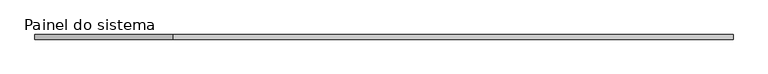
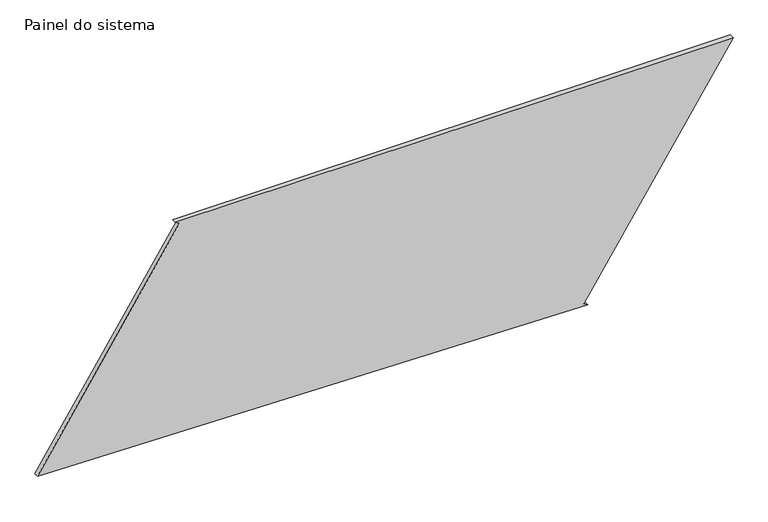
"""IFC4 building model written with IfcOpenShell, lengths in millimetres: plate geometry, Painel do sistema : Envidraçado."""

from ifc_helpers import new_model, si_unit, frame, origin, place, context, project, spatial, polyline, outline, extrude, source, transform, mapped, element, save


def painel_do_sistema_85665295(model_context):
    return source(origin(), model_context, "Body", "SweptSolid", [
        extrude(outline(polyline([(0.0, 1103.8254654), (13.6354654, 1082.8713707), (1262.5226251, 1895.5601522), (1262.5226251, -1143.9757701), (1248.8871597, -1123.0216755), (61.7003719, -1895.5601522), (0.0, 1103.8254654)])), frame((0.0, 24.5, 0.0), z_axis=(0.0, 1.0, 0.0), x_axis=(0.0, 0.0, 1.0)), (0.0, 0.0, 1.0), 25.0),
    ])


if __name__ == "__main__":
    model = new_model("IFC4")
    model_context = context("Model", 3, world=origin())
    ifc_project = project(units=[si_unit("LENGTHUNIT", "METRE", prefix="MILLI")], contexts=[model_context])
    site = spatial("IfcSite", under=ifc_project)
    building = spatial("IfcBuilding", under=site)
    placement = place(None, origin())
    painel_do_sistema_shape = painel_do_sistema_85665295(model_context)
    element("IfcPlate", 1, ObjectType="Painel do sistema : Envidraçado", at=placement, inside=building, context=model_context, shape_type="MappedRepresentation", body=[
        mapped(painel_do_sistema_shape, transform((0.0, 0.0, 0.0), x_axis=(1.0, 0.0, 0.0), y_axis=(0.0, 1.0, 0.0), z_axis=(0.0, 0.0, 1.0))),
    ])
    save(model, "model.ifc")

# Revit data of these elements
# Type "Painel do sistema : Envidraçado"
#   Construction Type Id = "GSP4R"
#   Analytic Construction = "Vidraça única Pilkington 1/8 pol"
#   Visual Light Transmittance = 0.9
#   Solar Heat Gain Coefficient = 0.86
#   Heat Transfer Coefficient (U) = 6.7069 W/(m²·K)
# Element 1 (IfcPlate, "Painel do sistema : Envidraçado")
#   Materials on its faces: "Vidro"
# Materials
#   "Vidro": class "Vidro", colour RGB 0 128 192, transparency 0.9, Description = "Vidro de sílica", Cost = 0
